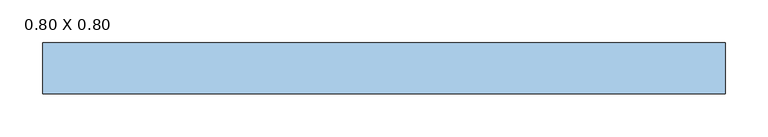
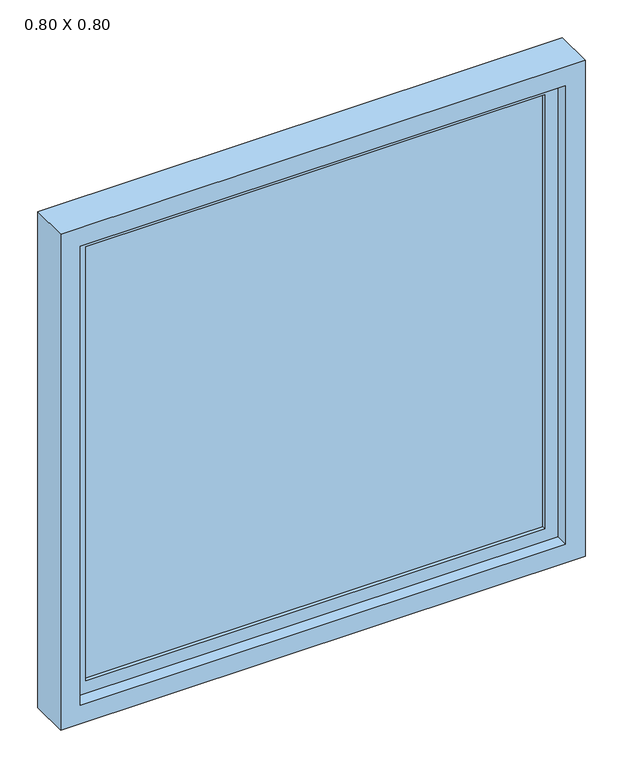
"""IFC4 building model written with IfcOpenShell, lengths in millimetres: window geometry, .CC_ND 300_MAXIM-AR : 0.80 X 0.80."""

import ifcopenshell
import ifcopenshell.guid

model = None  # the IFC model being written
_history = None  # IfcOwnerHistory: only IFC2X3 demands one
_inside = {}  # id of a spatial element -> (the spatial element, [elements in it])
_under = {}  # id of a project, library or spatial element -> (it, [spatial elements below it])
_declared = {}  # id of a project -> (the project, [libraries it declares])
_typed = {}  # id of a type object -> (the type object, [elements of that type])
_made_of = {}  # id of a material, layer set ... -> (it, [elements and type objects made of it])


def new_model(schema):
    """Start an empty IFC model of exactly this schema.

    Asked for "IFC4X3", IfcOpenShell would pick the latest addendum, in which some entities
    have other attributes; the version numbers below select the first issue.
    IFC2X3 requires an IfcOwnerHistory on every rooted entity: one is made here for all.
    """
    global model, _history
    if schema == "IFC4X3":
        model = ifcopenshell.file(schema_version=(4, 3, 0, 0))
    else:
        model = ifcopenshell.file(schema=schema)
    _inside.clear()
    _under.clear()
    _declared.clear()
    _typed.clear()
    _made_of.clear()
    _history = None
    if model.schema == "IFC2X3":
        org = make("IfcOrganization", Name="unknown")
        user = make(
            "IfcPersonAndOrganization",
            ThePerson=make("IfcPerson", FamilyName="unknown"),
            TheOrganization=org,
        )
        app = make(
            "IfcApplication",
            ApplicationDeveloper=org,
            Version="unknown",
            ApplicationFullName="unknown",
            ApplicationIdentifier="unknown",
        )
        _history = make(
            "IfcOwnerHistory",
            OwningUser=user,
            OwningApplication=app,
            ChangeAction="ADDED",
            CreationDate=0,
        )
    return model


def make(cls, **values):
    """One entity of the class cls with the attributes given. An attribute that is None is left unset."""
    return model.create_entity(
        cls, **{name: value for name, value in values.items() if value is not None}
    )


def rooted(cls, **values):
    """An entity with a GlobalId (a new one), such as an element, a storey or a relation."""
    return make(cls, GlobalId=ifcopenshell.guid.new(), OwnerHistory=_history, **values)


def si_unit(unit_type, name, prefix=None):
    """IfcSIUnit, for example si_unit("LENGTHUNIT", "METRE", prefix="MILLI")."""
    return make("IfcSIUnit", UnitType=unit_type, Prefix=prefix, Name=name)


def assignment(units):
    """IfcUnitAssignment: the units of a project."""
    return None if units is None else make("IfcUnitAssignment", Units=units)


def point(xyz):
    """IfcCartesianPoint."""
    return None if xyz is None else make("IfcCartesianPoint", Coordinates=xyz)


def direction(xyz):
    """IfcDirection."""
    return None if xyz is None else make("IfcDirection", DirectionRatios=xyz)


def frame(location, z_axis=None, x_axis=None):
    """IfcAxis2Placement3D, a coordinate frame: its origin and axes. An axis left out is left unset."""
    return make(
        "IfcAxis2Placement3D",
        Location=point(location),
        Axis=direction(z_axis),
        RefDirection=direction(x_axis),
    )


def origin():
    """The frame at (0, 0, 0) with its axes left unset."""
    return frame((0.0, 0.0, 0.0))


def place(relative_to, where):
    """IfcLocalPlacement: puts the frame where relative to a parent placement (None: the world)."""
    return make(
        "IfcLocalPlacement", PlacementRelTo=relative_to, RelativePlacement=where
    )


def context(
    kind, dimensions, precision=None, world=None, true_north=None, identifier=None
):
    """IfcGeometricRepresentationContext, for example the 3D "Model" context."""
    return make(
        "IfcGeometricRepresentationContext",
        ContextIdentifier=identifier,
        ContextType=kind,
        CoordinateSpaceDimension=dimensions,
        Precision=precision,
        WorldCoordinateSystem=world,
        TrueNorth=true_north,
    )


def project(units=None, contexts=None):
    """IfcProject with its units and contexts."""
    return rooted(
        "IfcProject",
        Name="project",
        RepresentationContexts=contexts,
        UnitsInContext=assignment(units),
    )


def spatial(cls, under=None, at=None, **own):
    """A site, building, storey or space (cls), placed at a placement, below another one or the project."""
    s = rooted(cls, ObjectPlacement=at, **own)
    if under is not None:
        _under.setdefault(under.id(), (under, []))[1].append(s)
    return s


def polyline(points):
    """IfcPolyline through the points."""
    return make("IfcPolyline", Points=[point(p) for p in points])


def outline(outer, holes=None, kind="AREA"):
    """IfcArbitraryClosedProfileDef: a profile drawn as a closed curve; with holes, ...WithVoids."""
    if holes is None:
        return make("IfcArbitraryClosedProfileDef", ProfileType=kind, OuterCurve=outer)
    return make(
        "IfcArbitraryProfileDefWithVoids",
        ProfileType=kind,
        OuterCurve=outer,
        InnerCurves=holes,
    )


def extrude(swept, where, along, depth):
    """IfcExtrudedAreaSolid: the profile swept, set in the frame where, extruded along a direction by depth."""
    return make(
        "IfcExtrudedAreaSolid",
        SweptArea=swept,
        Position=where,
        ExtrudedDirection=direction(along),
        Depth=depth,
    )


def shape(context_of_items, identifier, shape_type, items):
    """IfcShapeRepresentation: the items that make up one representation, for example the "Body"."""
    return make(
        "IfcShapeRepresentation",
        ContextOfItems=context_of_items,
        RepresentationIdentifier=identifier,
        RepresentationType=shape_type,
        Items=items,
    )


def source(mapping_origin, context_of_items, identifier, shape_type, items):
    """IfcRepresentationMap: a shape defined once, which mapped items show again and again."""
    return make(
        "IfcRepresentationMap",
        MappingOrigin=mapping_origin,
        MappedRepresentation=shape(context_of_items, identifier, shape_type, items),
    )


def transform(
    local_origin,
    x_axis=None,
    y_axis=None,
    z_axis=None,
    scale=None,
    scale2=None,
    scale3=None,
    uniform=True,
):
    """IfcCartesianTransformationOperator3D, or its non-uniform kind. x_axis, y_axis, z_axis: its Axis1, 2, 3."""
    if uniform:
        return make(
            "IfcCartesianTransformationOperator3D",
            Axis1=direction(x_axis),
            Axis2=direction(y_axis),
            LocalOrigin=point(local_origin),
            Scale=scale,
            Axis3=direction(z_axis),
        )
    return make(
        "IfcCartesianTransformationOperator3DnonUniform",
        Axis1=direction(x_axis),
        Axis2=direction(y_axis),
        LocalOrigin=point(local_origin),
        Scale=scale,
        Axis3=direction(z_axis),
        Scale2=scale2,
        Scale3=scale3,
    )


def mapped(mapping_source, mapping_target):
    """IfcMappedItem: shows the shape of a source again, moved by a transform."""
    return make(
        "IfcMappedItem", MappingSource=mapping_source, MappingTarget=mapping_target
    )


def made_of(thing, what):
    """Note that an element or type object is made of a material, layer set ...; save() writes the relation."""
    if what is not None:
        _made_of.setdefault(what.id(), (what, []))[1].append(thing)
    return thing


def element(
    cls,
    number,
    at=None,
    inside=None,
    cuts=None,
    type_object=None,
    material=None,
    context=None,
    identifier="Body",
    shape_type=None,
    held_by="IfcProductDefinitionShape",
    body=None,
    shapes=None,
    **own,
):
    """One element of the class cls, such as IfcWall. Its Tag is "e" and its number.

    at: its placement. inside: the storey or other place that contains it. cuts: it is an
    opening in that element (IfcRelVoidsElement). A single representation is given by context,
    identifier, shape_type and body (its items); several are given by shapes. held_by: the class
    of the entity that holds the representations. save() writes the other relations.
    """
    e = rooted(cls, Tag="e%d" % number, ObjectPlacement=at, **own)
    if body is not None:
        shapes = [shape(context, identifier, shape_type, body)]
    if shapes is not None:
        e.Representation = make(held_by, Representations=shapes)
    if inside is not None:
        _inside.setdefault(inside.id(), (inside, []))[1].append(e)
    if cuts is not None:
        rooted(
            "IfcRelVoidsElement", RelatingBuildingElement=cuts, RelatedOpeningElement=e
        )
    if type_object is not None:
        _typed.setdefault(type_object.id(), (type_object, []))[1].append(e)
    return made_of(e, material)


def aggregate(whole, parts):
    """IfcRelAggregates: a whole, such as a stair, and the parts it consists of."""
    return rooted("IfcRelAggregates", RelatingObject=whole, RelatedObjects=parts)


def save(model, path):
    """Write the relations noted so far, then the file.

    IfcRelAggregates (storeys below a building ...), IfcRelContainedInSpatialStructure (elements
    in a storey), IfcRelDefinesByType, IfcRelAssociatesMaterial and IfcRelDeclares: one each for
    every whole, place, type object, material and project.
    """
    for whole, parts in _under.values():
        aggregate(whole, parts)
    for where, things in _inside.values():
        rooted(
            "IfcRelContainedInSpatialStructure",
            RelatedElements=things,
            RelatingStructure=where,
        )
    for kind, things in _typed.values():
        rooted("IfcRelDefinesByType", RelatedObjects=things, RelatingType=kind)
    for what, things in _made_of.values():
        rooted("IfcRelAssociatesMaterial", RelatedObjects=things, RelatingMaterial=what)
    for by, libraries in _declared.values():
        rooted("IfcRelDeclares", RelatingContext=by, RelatedDefinitions=libraries)
    model.write(path)


def window_0_80_x_0_80_067849bc(model_context):
    return source(origin(), model_context, "Body", "SweptSolid", [
        extrude(outline(polyline([(-350.0, -4.0), (-350.0, 4.0), (350.0, 4.0), (350.0, -4.0), (-350.0, -4.0)])), frame((0.0, 0.0, 1550.0), z_axis=(0.0, 0.0, 1.0), x_axis=(1.0, 0.0, 0.0)), (0.0, 0.0, 1.0), 700.0),
        extrude(outline(polyline([(1530.0, 370.0), (2270.0, 370.0), (2270.0, -370.0), (1530.0, -370.0), (1530.0, 370.0)]), holes=[polyline([(2250.0, 350.0), (1550.0, 350.0), (1550.0, -350.0), (2250.0, -350.0), (2250.0, 350.0)])]), frame((0.0, -10.0, 0.0), z_axis=(0.0, 1.0, 0.0), x_axis=(0.0, 0.0, 1.0)), (0.0, 0.0, 1.0), 20.0),
        extrude(outline(polyline([(1500.0, 400.0), (2300.0, 400.0), (2300.0, -400.0), (1500.0, -400.0), (1500.0, 400.0)]), holes=[polyline([(2270.0, 370.0), (1530.0, 370.0), (1530.0, -370.0), (2270.0, -370.0), (2270.0, 370.0)])]), frame((0.0, -30.0, 0.0), z_axis=(0.0, 1.0, 0.0), x_axis=(0.0, 0.0, 1.0)), (0.0, 0.0, 1.0), 60.0),
    ])


if __name__ == "__main__":
    model = new_model("IFC4")
    model_context = context("Model", 3, world=origin())
    ifc_project = project(units=[si_unit("LENGTHUNIT", "METRE", prefix="MILLI")], contexts=[model_context])
    site = spatial("IfcSite", under=ifc_project)
    building = spatial("IfcBuilding", under=site)
    placement = place(None, origin())
    window_0_80_x_0_80_shape = window_0_80_x_0_80_067849bc(model_context)
    element("IfcWindow", 1, ObjectType=".CC_ND 300_MAXIM-AR : 0.80 X 0.80", at=placement, inside=building, context=model_context, shape_type="MappedRepresentation", body=[
        mapped(window_0_80_x_0_80_shape, transform((0.0, 0.0, 0.0), x_axis=(1.0, 0.0, 0.0), y_axis=(0.0, 1.0, 0.0), z_axis=(0.0, 0.0, 1.0))),
    ])
    save(model, "model.ifc")

# Revit data of these elements
# Type ".CC_ND 300_MAXIM-AR : 0.80 X 0.80"
#   Type Mark = "65"
#   Largura Painel [instance default] = 0.02 m
#   Largura Esquadria [instance default] = 0.06 m
#   Espessura Vidro [instance default] = 0.008 m
#   Espessura Painel [instance default] = 0.02 m
#   Espessura Esquadria [instance default] = 0.03 m
#   Height = 0.80 m
#   Altura-padrão do peitoril = 1.50 m
#   Width = 0.80 m
#   Vidro = .VIDRO GENÉRICO
#   Esquadria = .ALUMÍNIO COM PINTURA ELETROSTÁTICA BRANCA
#   Wall Closure = (empty or 0)
# Element 1 (IfcWindow, ".CC_ND 300_MAXIM-AR : 0.80 X 0.80")
#   Materials on its faces: ".ALUMÍNIO COM PINTURA ELETROSTÁTICA BRANCA", ".VIDRO GENÉRICO"
# Materials
#   ".VIDRO GENÉRICO": class ".CC_VIDRO", colour RGB 0 128 192, transparency 0.9, Description = "Vidro comum", Cost = 0
#   ".ALUMÍNIO COM PINTURA ELETROSTÁTICA BRANCA": class "CC_METAIS", colour RGB 241 241 241, transparency 0, Cost = 0
